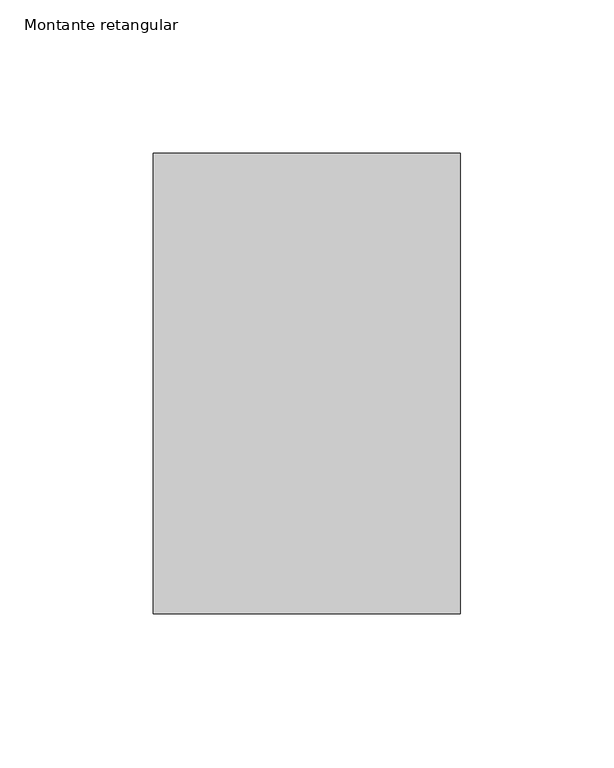
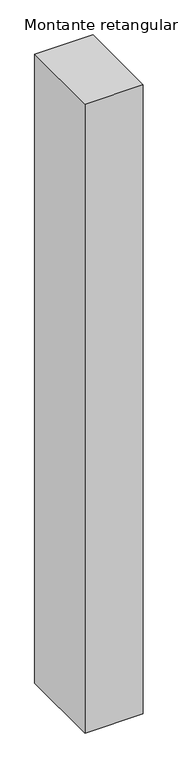
"""IFC4 building model written with IfcOpenShell, lengths in millimetres: member geometry, Montante retangular : CC_100 X 150  mm."""

from ifc_helpers import new_model, si_unit, frame, origin, place, context, project, spatial, polyline, outline, extrude, source, transform, mapped, element, save


def montante_retangular_d0ec09bd(model_context):
    return source(origin(), model_context, "Body", "SweptSolid", [
        extrude(outline(polyline([(50.0, 75.0), (50.0, -75.0), (-50.0, -75.0), (-50.0, 75.0), (50.0, 75.0)])), frame((0.0, 0.0, -1143.7500002), z_axis=(0.0, 0.0, 1.0), x_axis=(1.0, 0.0, 0.0)), (0.0, 0.0, 1.0), 1143.7500002),
    ])


if __name__ == "__main__":
    model = new_model("IFC4")
    model_context = context("Model", 3, world=origin())
    ifc_project = project(units=[si_unit("LENGTHUNIT", "METRE", prefix="MILLI")], contexts=[model_context])
    site = spatial("IfcSite", under=ifc_project)
    building = spatial("IfcBuilding", under=site)
    placement = place(None, origin())
    montante_retangular_shape = montante_retangular_d0ec09bd(model_context)
    element("IfcMember", 1, ObjectType="Montante retangular : CC_100 X 150  mm", at=placement, inside=building, context=model_context, shape_type="MappedRepresentation", body=[
        mapped(montante_retangular_shape, transform((0.0, 0.0, 0.0), x_axis=(1.0, 0.0, 0.0), y_axis=(0.0, 1.0, 0.0), z_axis=(0.0, 0.0, 1.0))),
    ])
    save(model, "model.ifc")

# Revit data of these elements
# Type "Montante retangular : CC_100 X 150  mm"
#   built-in parameter 1007304 = 0.492126 (stored number, unit not read)
#   built-in parameter 1007301 = 0.164042 (stored number, unit not read)
#   built-in parameter 1007300 = 0.164042 (stored number, unit not read)
# Element 1 (IfcMember, "Montante retangular : CC_100 X 150  mm")
#   Materials on its faces: ".ALUMÍNIO"
# Materials
#   ".ALUMÍNIO": class "CC_METAIS", colour RGB 244 244 244, transparency 0, Description = "Material alumínio", Cost = 0
